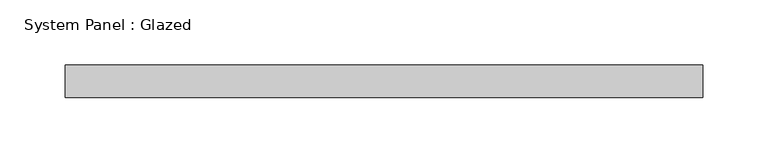
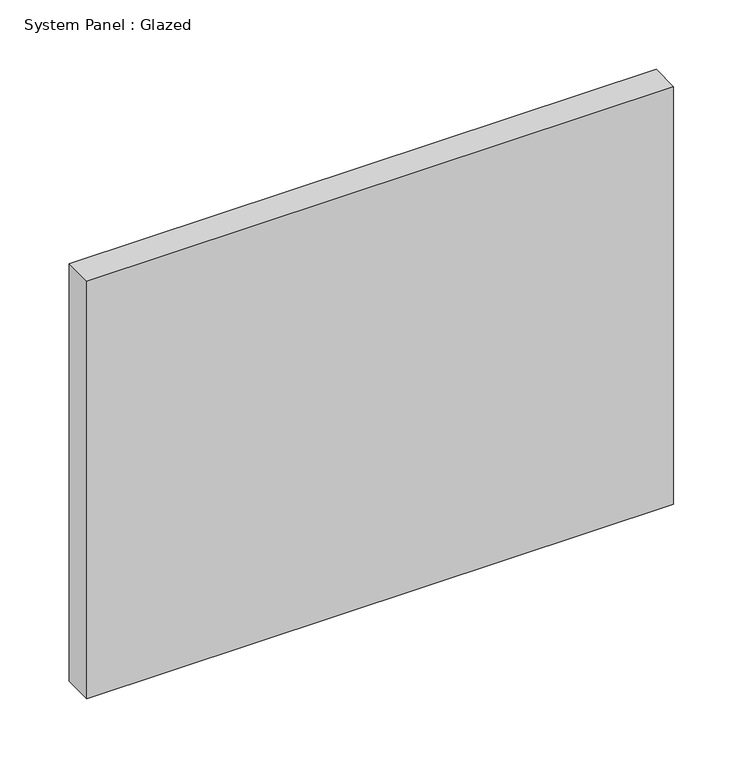
"""IFC4 building model written with IfcOpenShell, lengths in millimetres: plate geometry, System Panel : Glazed."""

import ifcopenshell
import ifcopenshell.guid

model = None  # the IFC model being written
_history = None  # IfcOwnerHistory: only IFC2X3 demands one
_inside = {}  # id of a spatial element -> (the spatial element, [elements in it])
_under = {}  # id of a project, library or spatial element -> (it, [spatial elements below it])
_declared = {}  # id of a project -> (the project, [libraries it declares])
_typed = {}  # id of a type object -> (the type object, [elements of that type])
_made_of = {}  # id of a material, layer set ... -> (it, [elements and type objects made of it])


def new_model(schema):
    """Start an empty IFC model of exactly this schema.

    Asked for "IFC4X3", IfcOpenShell would pick the latest addendum, in which some entities
    have other attributes; the version numbers below select the first issue.
    IFC2X3 requires an IfcOwnerHistory on every rooted entity: one is made here for all.
    """
    global model, _history
    if schema == "IFC4X3":
        model = ifcopenshell.file(schema_version=(4, 3, 0, 0))
    else:
        model = ifcopenshell.file(schema=schema)
    _inside.clear()
    _under.clear()
    _declared.clear()
    _typed.clear()
    _made_of.clear()
    _history = None
    if model.schema == "IFC2X3":
        org = make("IfcOrganization", Name="unknown")
        user = make(
            "IfcPersonAndOrganization",
            ThePerson=make("IfcPerson", FamilyName="unknown"),
            TheOrganization=org,
        )
        app = make(
            "IfcApplication",
            ApplicationDeveloper=org,
            Version="unknown",
            ApplicationFullName="unknown",
            ApplicationIdentifier="unknown",
        )
        _history = make(
            "IfcOwnerHistory",
            OwningUser=user,
            OwningApplication=app,
            ChangeAction="ADDED",
            CreationDate=0,
        )
    return model


def make(cls, **values):
    """One entity of the class cls with the attributes given. An attribute that is None is left unset."""
    return model.create_entity(
        cls, **{name: value for name, value in values.items() if value is not None}
    )


def rooted(cls, **values):
    """An entity with a GlobalId (a new one), such as an element, a storey or a relation."""
    return make(cls, GlobalId=ifcopenshell.guid.new(), OwnerHistory=_history, **values)


def si_unit(unit_type, name, prefix=None):
    """IfcSIUnit, for example si_unit("LENGTHUNIT", "METRE", prefix="MILLI")."""
    return make("IfcSIUnit", UnitType=unit_type, Prefix=prefix, Name=name)


def assignment(units):
    """IfcUnitAssignment: the units of a project."""
    return None if units is None else make("IfcUnitAssignment", Units=units)


def point(xyz):
    """IfcCartesianPoint."""
    return None if xyz is None else make("IfcCartesianPoint", Coordinates=xyz)


def direction(xyz):
    """IfcDirection."""
    return None if xyz is None else make("IfcDirection", DirectionRatios=xyz)


def frame(location, z_axis=None, x_axis=None):
    """IfcAxis2Placement3D, a coordinate frame: its origin and axes. An axis left out is left unset."""
    return make(
        "IfcAxis2Placement3D",
        Location=point(location),
        Axis=direction(z_axis),
        RefDirection=direction(x_axis),
    )


def origin():
    """The frame at (0, 0, 0) with its axes left unset."""
    return frame((0.0, 0.0, 0.0))


def origin_with_axes():
    """The frame at (0, 0, 0) with the z axis (0, 0, 1) and the x axis (1, 0, 0) written out."""
    return frame((0.0, 0.0, 0.0), z_axis=(0.0, 0.0, 1.0), x_axis=(1.0, 0.0, 0.0))


def place(relative_to, where):
    """IfcLocalPlacement: puts the frame where relative to a parent placement (None: the world)."""
    return make(
        "IfcLocalPlacement", PlacementRelTo=relative_to, RelativePlacement=where
    )


def context(
    kind, dimensions, precision=None, world=None, true_north=None, identifier=None
):
    """IfcGeometricRepresentationContext, for example the 3D "Model" context."""
    return make(
        "IfcGeometricRepresentationContext",
        ContextIdentifier=identifier,
        ContextType=kind,
        CoordinateSpaceDimension=dimensions,
        Precision=precision,
        WorldCoordinateSystem=world,
        TrueNorth=true_north,
    )


def project(units=None, contexts=None):
    """IfcProject with its units and contexts."""
    return rooted(
        "IfcProject",
        Name="project",
        RepresentationContexts=contexts,
        UnitsInContext=assignment(units),
    )


def spatial(cls, under=None, at=None, **own):
    """A site, building, storey or space (cls), placed at a placement, below another one or the project."""
    s = rooted(cls, ObjectPlacement=at, **own)
    if under is not None:
        _under.setdefault(under.id(), (under, []))[1].append(s)
    return s


def polyline(points):
    """IfcPolyline through the points."""
    return make("IfcPolyline", Points=[point(p) for p in points])


def outline(outer, holes=None, kind="AREA"):
    """IfcArbitraryClosedProfileDef: a profile drawn as a closed curve; with holes, ...WithVoids."""
    if holes is None:
        return make("IfcArbitraryClosedProfileDef", ProfileType=kind, OuterCurve=outer)
    return make(
        "IfcArbitraryProfileDefWithVoids",
        ProfileType=kind,
        OuterCurve=outer,
        InnerCurves=holes,
    )


def extrude(swept, where, along, depth):
    """IfcExtrudedAreaSolid: the profile swept, set in the frame where, extruded along a direction by depth."""
    return make(
        "IfcExtrudedAreaSolid",
        SweptArea=swept,
        Position=where,
        ExtrudedDirection=direction(along),
        Depth=depth,
    )


def shape(context_of_items, identifier, shape_type, items):
    """IfcShapeRepresentation: the items that make up one representation, for example the "Body"."""
    return make(
        "IfcShapeRepresentation",
        ContextOfItems=context_of_items,
        RepresentationIdentifier=identifier,
        RepresentationType=shape_type,
        Items=items,
    )


def source(mapping_origin, context_of_items, identifier, shape_type, items):
    """IfcRepresentationMap: a shape defined once, which mapped items show again and again."""
    return make(
        "IfcRepresentationMap",
        MappingOrigin=mapping_origin,
        MappedRepresentation=shape(context_of_items, identifier, shape_type, items),
    )


def transform(
    local_origin,
    x_axis=None,
    y_axis=None,
    z_axis=None,
    scale=None,
    scale2=None,
    scale3=None,
    uniform=True,
):
    """IfcCartesianTransformationOperator3D, or its non-uniform kind. x_axis, y_axis, z_axis: its Axis1, 2, 3."""
    if uniform:
        return make(
            "IfcCartesianTransformationOperator3D",
            Axis1=direction(x_axis),
            Axis2=direction(y_axis),
            LocalOrigin=point(local_origin),
            Scale=scale,
            Axis3=direction(z_axis),
        )
    return make(
        "IfcCartesianTransformationOperator3DnonUniform",
        Axis1=direction(x_axis),
        Axis2=direction(y_axis),
        LocalOrigin=point(local_origin),
        Scale=scale,
        Axis3=direction(z_axis),
        Scale2=scale2,
        Scale3=scale3,
    )


def mapped(mapping_source, mapping_target):
    """IfcMappedItem: shows the shape of a source again, moved by a transform."""
    return make(
        "IfcMappedItem", MappingSource=mapping_source, MappingTarget=mapping_target
    )


def made_of(thing, what):
    """Note that an element or type object is made of a material, layer set ...; save() writes the relation."""
    if what is not None:
        _made_of.setdefault(what.id(), (what, []))[1].append(thing)
    return thing


def element(
    cls,
    number,
    at=None,
    inside=None,
    cuts=None,
    type_object=None,
    material=None,
    context=None,
    identifier="Body",
    shape_type=None,
    held_by="IfcProductDefinitionShape",
    body=None,
    shapes=None,
    **own,
):
    """One element of the class cls, such as IfcWall. Its Tag is "e" and its number.

    at: its placement. inside: the storey or other place that contains it. cuts: it is an
    opening in that element (IfcRelVoidsElement). A single representation is given by context,
    identifier, shape_type and body (its items); several are given by shapes. held_by: the class
    of the entity that holds the representations. save() writes the other relations.
    """
    e = rooted(cls, Tag="e%d" % number, ObjectPlacement=at, **own)
    if body is not None:
        shapes = [shape(context, identifier, shape_type, body)]
    if shapes is not None:
        e.Representation = make(held_by, Representations=shapes)
    if inside is not None:
        _inside.setdefault(inside.id(), (inside, []))[1].append(e)
    if cuts is not None:
        rooted(
            "IfcRelVoidsElement", RelatingBuildingElement=cuts, RelatedOpeningElement=e
        )
    if type_object is not None:
        _typed.setdefault(type_object.id(), (type_object, []))[1].append(e)
    return made_of(e, material)


def aggregate(whole, parts):
    """IfcRelAggregates: a whole, such as a stair, and the parts it consists of."""
    return rooted("IfcRelAggregates", RelatingObject=whole, RelatedObjects=parts)


def save(model, path):
    """Write the relations noted so far, then the file.

    IfcRelAggregates (storeys below a building ...), IfcRelContainedInSpatialStructure (elements
    in a storey), IfcRelDefinesByType, IfcRelAssociatesMaterial and IfcRelDeclares: one each for
    every whole, place, type object, material and project.
    """
    for whole, parts in _under.values():
        aggregate(whole, parts)
    for where, things in _inside.values():
        rooted(
            "IfcRelContainedInSpatialStructure",
            RelatedElements=things,
            RelatingStructure=where,
        )
    for kind, things in _typed.values():
        rooted("IfcRelDefinesByType", RelatedObjects=things, RelatingType=kind)
    for what, things in _made_of.values():
        rooted("IfcRelAssociatesMaterial", RelatedObjects=things, RelatingMaterial=what)
    for by, libraries in _declared.values():
        rooted("IfcRelDeclares", RelatingContext=by, RelatedDefinitions=libraries)
    model.write(path)


def system_panel_glazed_d9052cd5(model_context):
    return source(origin(), model_context, "Body", "SweptSolid", [
        extrude(outline(polyline([(243.9393939, 24.5), (-243.9393939, 24.5), (-243.9393939, 49.5), (243.9393939, 49.5), (243.9393939, 24.5)])), origin_with_axes(), (0.0, 0.0, 1.0), 366.6666667),
    ])


if __name__ == "__main__":
    model = new_model("IFC4")
    model_context = context("Model", 3, world=origin())
    ifc_project = project(units=[si_unit("LENGTHUNIT", "METRE", prefix="MILLI")], contexts=[model_context])
    site = spatial("IfcSite", under=ifc_project)
    building = spatial("IfcBuilding", under=site)
    placement = place(None, origin())
    system_panel_glazed_shape = system_panel_glazed_d9052cd5(model_context)
    element("IfcPlate", 1, ObjectType="System Panel : Glazed", at=placement, inside=building, context=model_context, shape_type="MappedRepresentation", body=[
        mapped(system_panel_glazed_shape, transform((0.0, 0.0, 0.0), x_axis=(1.0, 0.0, 0.0), y_axis=(0.0, 1.0, 0.0), z_axis=(0.0, 0.0, 1.0))),
    ])
    save(model, "model.ifc")

# Revit data of these elements
# Element 1 (IfcPlate, "System Panel : Glazed")
#   Materials on its faces: "Glass"
# Materials
#   "Glass": class "Glass", colour RGB 218 227 224, transparency 0.85, Description = "Soda Lime Glass", Cost = 0
